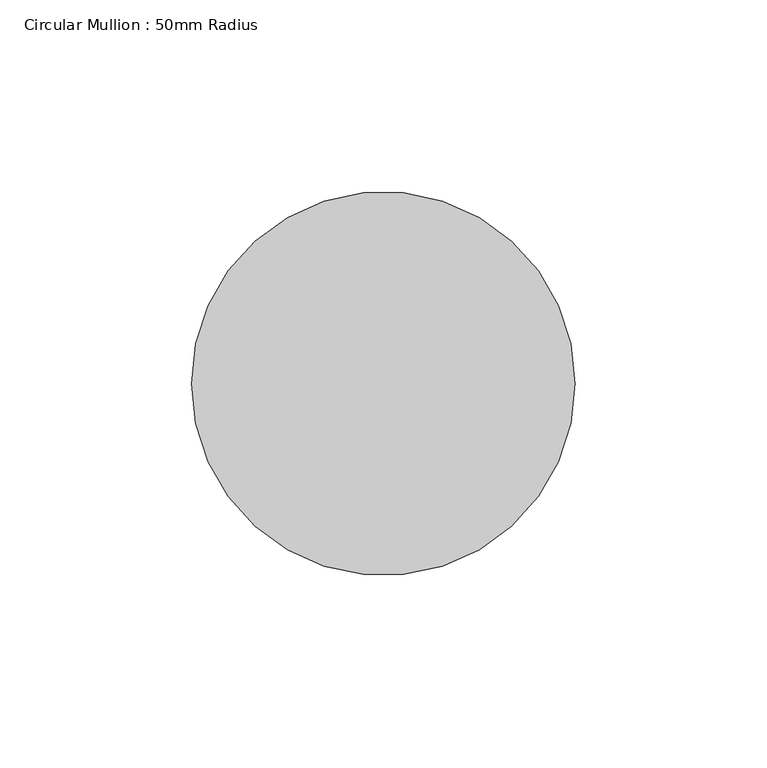
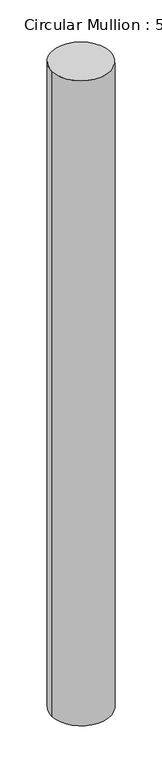
"""IFC4 building model written with IfcOpenShell, lengths in millimetres: member geometry, Circular Mullion : 50mm Radius."""

from ifc_helpers import new_model, si_unit, point, frame, origin, origin_2d, place, context, project, spatial, circle_curve, trimmed, segment, composite_curve, outline, extrude, source, transform, mapped, element, save


def circular_mullion_50mm_radius_0ee71593(model_context):
    return source(origin(), model_context, "Body", "SweptSolid", [
        extrude(outline(composite_curve([segment(trimmed(circle_curve(origin_2d(), 50.0), [point((50.0, 0.0))], [point((-50.0, 0.0))], False, "CARTESIAN"), True, "CONTINUOUS"), segment(trimmed(circle_curve(origin_2d(), 50.0), [point((-50.0, 0.0))], [point((50.0, 0.0))], False, "CARTESIAN"), True, "CONTINUOUS")], self_intersect=False)), frame((0.0, 0.0, -1162.0262438), z_axis=(0.0, 0.0, 1.0), x_axis=(1.0, 0.0, 0.0)), (0.0, 0.0, 1.0), 1162.0262438),
    ])


if __name__ == "__main__":
    model = new_model("IFC4")
    model_context = context("Model", 3, world=origin())
    ifc_project = project(units=[si_unit("LENGTHUNIT", "METRE", prefix="MILLI")], contexts=[model_context])
    site = spatial("IfcSite", under=ifc_project)
    building = spatial("IfcBuilding", under=site)
    placement = place(None, origin())
    circular_mullion_50mm_radius_shape = circular_mullion_50mm_radius_0ee71593(model_context)
    element("IfcMember", 1, ObjectType="Circular Mullion : 50mm Radius", at=placement, inside=building, context=model_context, shape_type="MappedRepresentation", body=[
        mapped(circular_mullion_50mm_radius_shape, transform((0.0, 0.0, 0.0), x_axis=(1.0, 0.0, 0.0), y_axis=(0.0, 1.0, 0.0), z_axis=(0.0, 0.0, 1.0))),
    ])
    save(model, "model.ifc")

# Revit data of these elements
# Type "Circular Mullion : 50mm Radius"
#   built-in parameter 1007350 = 0.164042 (stored number, unit not read)
# Element 1 (IfcMember, "Circular Mullion : 50mm Radius")
#   Materials on its faces: "Aluminium"
# Materials
#   "Aluminium": class "Metal", colour RGB 247 247 247, transparency 0, Description = "Aluminium 6061", Cost = 0
